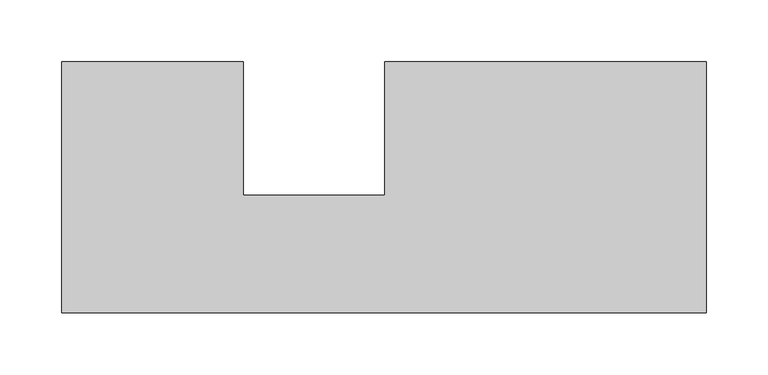
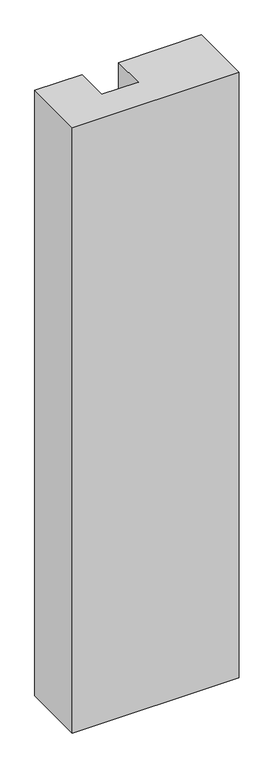
"""IFC4 building model written with IfcOpenShell, lengths in millimetres: proxy geometry, Generic Models 7:Generic Models 1:3:Generic Models 1:3 : Generic Models 7:Generic Models 1:305549:3:Generic Models 1:3:Generic Models 1:3 : Generic Models 7:Generic Models 1:305549:3 : Generic Models 7:Generic Models 1:3:Generic Models 1:3 : Generic Models 7:Generic Models 1:305549:301244:16 : Generic Models 7:Generic Models 1:3:Generic Models 1:3 : Generic Models 7:Generic Models 1:305549:3:Generic Models 1:3:Generic Models 1:3 : Generic Models 7:Generic Models 1:305549:3 : Generic Models 7:Generic Models 1:3:Generic Models 1:3 : Generic Models 7:Generic Models 1:305549:301244:308848."""

from ifc_helpers import new_model, si_unit, frame, origin, place, context, project, spatial, polyline, outline, extrude, source, transform, mapped, element, save


def generic_models_f43d386e(model_context):
    return source(origin(), model_context, "Body", "SweptSolid", [
        extrude(outline(polyline([(560512.7908247, -578905.4413841), (560627.0908247, -578905.4413841), (560627.0908247, -578797.4913841), (560887.4408247, -578797.4913841), (560887.4408247, -579000.6913841), (560365.6617239, -579000.6913841), (560365.6617239, -578797.4913841), (560512.7908247, -578797.4913841), (560512.7908247, -578905.4413841)])), frame((0.0, 0.0, 4133.81326), z_axis=(0.0, 0.0, 1.0), x_axis=(1.0, 0.0, 0.0)), (0.0, 0.0, 1.0), 2000.28674),
    ])


if __name__ == "__main__":
    model = new_model("IFC4")
    model_context = context("Model", 3, world=origin())
    ifc_project = project(units=[si_unit("LENGTHUNIT", "METRE", prefix="MILLI")], contexts=[model_context])
    site = spatial("IfcSite", under=ifc_project)
    building = spatial("IfcBuilding", under=site)
    placement = place(None, origin())
    generic_models_shape = generic_models_f43d386e(model_context)
    element("IfcBuildingElementProxy", 1, Name="Generic Models 7:Generic Models 1:3:Generic Models 1:3 : Generic Models 7:Generic Models 1:305549:3:Generic Models 1:3:Generic Models 1:3 : Generic Models 7:Generic Models 1:305549:3 : Generic Models 7:Generic Models 1:3:Generic Models 1:3 : Generic Models 7:Generic Models 1:305549:301244:16 : Generic Models 7:Generic Models 1:3:Generic Models 1:3 : Generic Models 7:Generic Models 1:305549:3:Generic Models 1:3:Generic Models 1:3 : Generic Models 7:Generic Models 1:305549:3 : Generic Models 7:Generic Models 1:3:Generic Models 1:3 : Generic Models 7:Generic Models 1:305549:301244:308848", ObjectType="Generic Models 7:Generic Models 1:3:Generic Models 1:3 : Generic Models 7:Generic Models 1:305549:3:Generic Models 1:3:Generic Models 1:3 : Generic Models 7:Generic Models 1:305549:3 : Generic Models 7:Generic Models 1:3:Generic Models 1:3 : Generic Models 7:Generic Models 1:305549:301244:16 : Generic Models 7:Generic Models 1:3:Generic Models 1:3 : Generic Models 7:Generic Models 1:305549:3:Generic Models 1:3:Generic Models 1:3 : Generic Models 7:Generic Models 1:305549:3 : Generic Models 7:Generic Models 1:3:Generic Models 1:3 : Generic Models 7:Generic Models 1:305549:301244:308848", at=placement, inside=building, context=model_context, shape_type="MappedRepresentation", body=[
        mapped(generic_models_shape, transform((0.0, 0.0, 0.0), x_axis=(1.0, 0.0, 0.0), y_axis=(0.0, 1.0, 0.0), z_axis=(0.0, 0.0, 1.0))),
    ])
    save(model, "model.ifc")

# Revit data of these elements
# Type "Generic Models 7:Generic Models 1:3:Generic Models 1:3 : Generic Models 7:Generic Models 1:305549:3:Generic Models 1:3:Generic Models 1:3 : Generic Models 7:Generic Models 1:305549:3 : Generic Models 7:Generic Models 1:3:Generic Models 1:3 : Generic Models 7:Generic Models 1:305549:301244:16 : Generic Models 7:Generic Models 1:3:Generic Models 1:3 : Generic Models 7:Generic Models 1:305549:3:Generic Models 1:3:Generic Models 1:3 : Generic Models 7:Generic Models 1:305549:3 : Generic Models 7:Generic Models 1:3:Generic Models 1:3 : Generic Models 7:Generic Models 1:305549:301244:308848"
#   NameOverride = "Generic Models 7:Generic Models 1:3:Generic Models 1:3 : Generic Models 7:Generic Models 1:305549:3:Generic Models 1:3:Generic Models 1:3 : Generic Models 7:Generic Models 1:305549:3 : Generic Models 7:Generic Models 1:3:Generic Models 1:3 : Generic Models 7:Generic Models 1:305549:301244:308848"
#   ObjectTypeOverride = "Generic Models 1:3:Generic Models 1:3 : Generic Models 7:Generic Models 1:305549:3 : Generic Models 7:Generic Models 1:3:Generic Models 1:3 : Generic Models 7:Generic Models 1:305549:301244"
#   Reference = "Generic Models 1"
#   Tag = "308848"
# Element 1 (IfcBuildingElementProxy, "Generic Models 7:Generic Models 1:3:Generic Models 1:3 : Generic Models 7:Generic Models 1:305549:3:Generic Models 1:3:Generic Models 1:3 : Generic Models 7:Generic Models 1:305549:3 : Generic Models 7:Generic Models 1:3:Generic Models 1:3 : Generic Models 7:Generic Models 1:305549:301244:16 : Generic Models 7:Generic Models 1:3:Generic Models 1:3 : Generic Models 7:Generic Models 1:305549:3:Generic Models 1:3:Generic Models 1:3 : Generic Models 7:Generic Models 1:305549:3 : Generic Models 7:Generic Models 1:3:Generic Models 1:3 : Generic Models 7:Generic Models 1:305549:301244:308848")
#   Materials on its faces: "FULL CAVITY CLASS A FIBERGLASS INSULATION WITH DURABLE VAPOR BARRIER (BLACK) LINER"
# Materials
#   "FULL CAVITY CLASS A FIBERGLASS INSULATION WITH DURABLE VAPOR BARRIER (BLACK) LINER": class "Unassigned", colour RGB 158 92 175, transparency 0, Cost = 0
